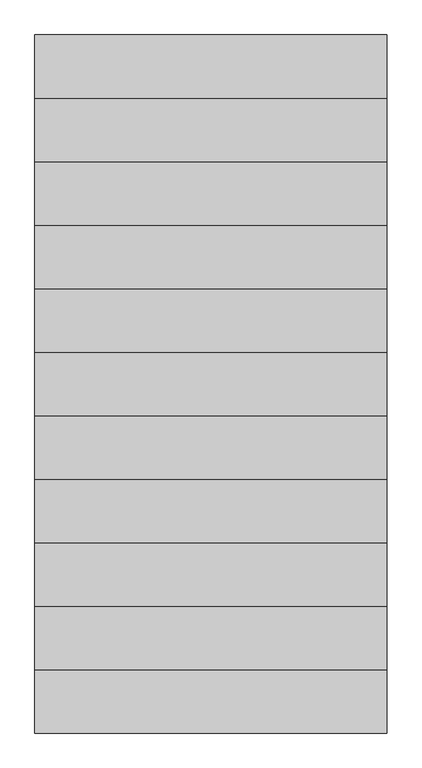
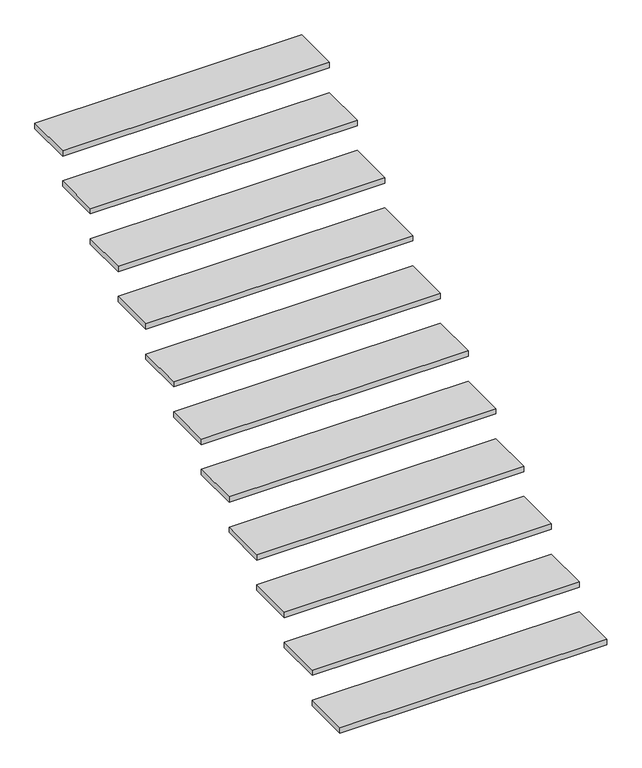
"""IFC4 building model written with IfcOpenShell, lengths in millimetres: stair flight geometry."""

from ifc_helpers import new_model, si_unit, frame, origin, place, context, project, spatial, polyline, outline, extrude, source, transform, mapped, element, save


def stair_flight_92cbd049(model_context):
    return source(origin(), model_context, "Body", "SweptSolid", [
        extrude(outline(polyline([(17005.3403387, 2217.6066446), (18505.3403387, 2217.6066446), (18505.3403387, 1947.6066446), (17005.3403387, 1947.6066446), (17005.3403387, 2217.6066446)])), frame((0.0, 0.0, 147.1208791), z_axis=(0.0, 0.0, 1.0), x_axis=(1.0, 0.0, 0.0)), (0.0, 0.0, 1.0), 32.0),
        extrude(outline(polyline([(17005.3403387, 2487.6066446), (18505.3403387, 2487.6066446), (18505.3403387, 2217.6066446), (17005.3403387, 2217.6066446), (17005.3403387, 2487.6066446)])), frame((0.0, 0.0, 326.2417582), z_axis=(0.0, 0.0, 1.0), x_axis=(1.0, 0.0, 0.0)), (0.0, 0.0, 1.0), 32.0),
        extrude(outline(polyline([(17005.3403387, 2757.6066446), (18505.3403387, 2757.6066446), (18505.3403387, 2487.6066446), (17005.3403387, 2487.6066446), (17005.3403387, 2757.6066446)])), frame((0.0, 0.0, 505.3626374), z_axis=(0.0, 0.0, 1.0), x_axis=(1.0, 0.0, 0.0)), (0.0, 0.0, 1.0), 32.0),
        extrude(outline(polyline([(17005.3403387, 3027.6066446), (18505.3403387, 3027.6066446), (18505.3403387, 2757.6066446), (17005.3403387, 2757.6066446), (17005.3403387, 3027.6066446)])), frame((0.0, 0.0, 684.4835165), z_axis=(0.0, 0.0, 1.0), x_axis=(1.0, 0.0, 0.0)), (0.0, 0.0, 1.0), 32.0),
        extrude(outline(polyline([(17005.3403387, 3297.6066446), (18505.3403387, 3297.6066446), (18505.3403387, 3027.6066446), (17005.3403387, 3027.6066446), (17005.3403387, 3297.6066446)])), frame((0.0, 0.0, 863.6043956), z_axis=(0.0, 0.0, 1.0), x_axis=(1.0, 0.0, 0.0)), (0.0, 0.0, 1.0), 32.0),
        extrude(outline(polyline([(17005.3403387, 3567.6066446), (18505.3403387, 3567.6066446), (18505.3403387, 3297.6066446), (17005.3403387, 3297.6066446), (17005.3403387, 3567.6066446)])), frame((0.0, 0.0, 1042.7252747), z_axis=(0.0, 0.0, 1.0), x_axis=(1.0, 0.0, 0.0)), (0.0, 0.0, 1.0), 32.0),
        extrude(outline(polyline([(17005.3403387, 3837.6066446), (18505.3403387, 3837.6066446), (18505.3403387, 3567.6066446), (17005.3403387, 3567.6066446), (17005.3403387, 3837.6066446)])), frame((0.0, 0.0, 1221.8461538), z_axis=(0.0, 0.0, 1.0), x_axis=(1.0, 0.0, 0.0)), (0.0, 0.0, 1.0), 32.0),
        extrude(outline(polyline([(17005.3403387, 4107.6066446), (18505.3403387, 4107.6066446), (18505.3403387, 3837.6066446), (17005.3403387, 3837.6066446), (17005.3403387, 4107.6066446)])), frame((0.0, 0.0, 1400.967033), z_axis=(0.0, 0.0, 1.0), x_axis=(1.0, 0.0, 0.0)), (0.0, 0.0, 1.0), 32.0),
        extrude(outline(polyline([(17005.3403387, 4377.6066446), (18505.3403387, 4377.6066446), (18505.3403387, 4107.6066446), (17005.3403387, 4107.6066446), (17005.3403387, 4377.6066446)])), frame((0.0, 0.0, 1580.0879121), z_axis=(0.0, 0.0, 1.0), x_axis=(1.0, 0.0, 0.0)), (0.0, 0.0, 1.0), 32.0),
        extrude(outline(polyline([(17005.3403387, 4647.6066446), (18505.3403387, 4647.6066446), (18505.3403387, 4377.6066446), (17005.3403387, 4377.6066446), (17005.3403387, 4647.6066446)])), frame((0.0, 0.0, 1759.2087912), z_axis=(0.0, 0.0, 1.0), x_axis=(1.0, 0.0, 0.0)), (0.0, 0.0, 1.0), 32.0),
        extrude(outline(polyline([(17005.3403387, 4917.6066446), (18505.3403387, 4917.6066446), (18505.3403387, 4647.6066446), (17005.3403387, 4647.6066446), (17005.3403387, 4917.6066446)])), frame((0.0, 0.0, 1938.3296703), z_axis=(0.0, 0.0, 1.0), x_axis=(1.0, 0.0, 0.0)), (0.0, 0.0, 1.0), 32.0),
    ])


if __name__ == "__main__":
    model = new_model("IFC4")
    model_context = context("Model", 3, world=origin())
    ifc_project = project(units=[si_unit("LENGTHUNIT", "METRE", prefix="MILLI")], contexts=[model_context])
    site = spatial("IfcSite", under=ifc_project)
    building = spatial("IfcBuilding", under=site)
    placement = place(None, origin())
    stair_flight_shape = stair_flight_92cbd049(model_context)
    element("IfcStairFlight", 1, at=placement, inside=building, context=model_context, shape_type="MappedRepresentation", body=[
        mapped(stair_flight_shape, transform((0.0, 0.0, 0.0), x_axis=(1.0, 0.0, 0.0), y_axis=(0.0, 1.0, 0.0), z_axis=(0.0, 0.0, 1.0))),
    ])
    save(model, "model.ifc")

# Revit data of these elements
# Element 1 (IfcStairFlight)
#   Materials on its faces: "철강"
# Materials
#   "철강": class "Generic", colour RGB 143 142 141, transparency 0, Description = "철골+가공조립+세우기", Cost = 0
